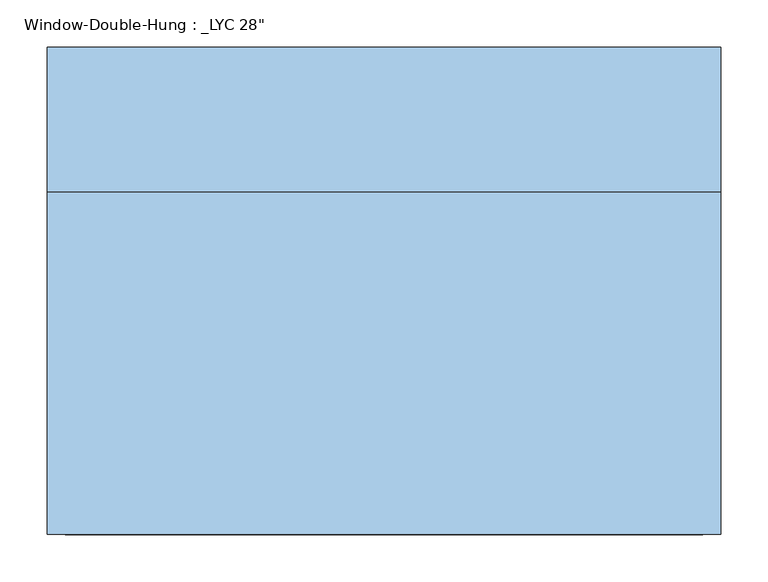
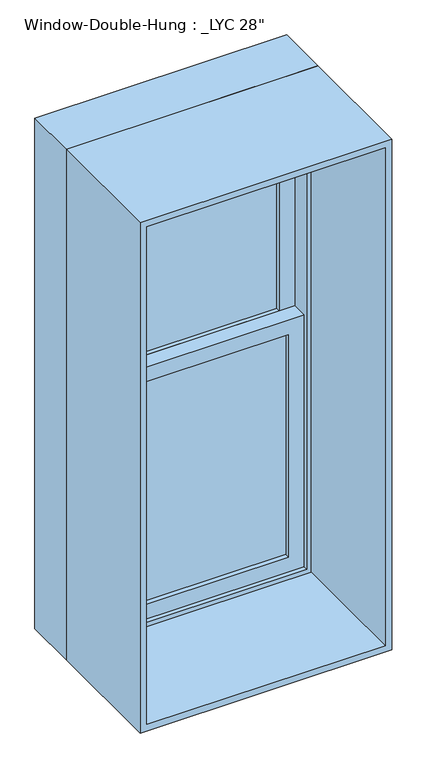
"""IFC4 building model written with IfcOpenShell, lengths in millimetres: window geometry."""

from ifc_helpers import new_model, si_unit, frame, origin, place, context, project, spatial, polyline, outline, extrude, source, transform, mapped, element, save


def window_246d4ddb(model_context):
    return source(origin(), model_context, "Body", "SweptSolid", [
        extrude(outline(polyline([(279.4, 158.75), (279.4, 152.4), (-279.4, 152.4), (-279.4, 158.75), (279.4, 158.75)])), frame((0.0, 0.0, 990.6), z_axis=(0.0, 0.0, 1.0), x_axis=(1.0, 0.0, 0.0)), (0.0, 0.0, 1.0), 663.575),
        extrude(outline(polyline([(-279.4, 146.05), (279.4, 146.05), (279.4, 139.7), (-279.4, 139.7), (-279.4, 146.05)])), frame((0.0, 0.0, 990.6), z_axis=(0.0, 0.0, 1.0), x_axis=(1.0, 0.0, 0.0)), (0.0, 0.0, 1.0), 663.575),
        extrude(outline(polyline([(279.4, 203.2), (279.4, 196.85), (-279.4, 196.85), (-279.4, 203.2), (279.4, 203.2)])), frame((0.0, 0.0, 1698.625), z_axis=(0.0, 0.0, 1.0), x_axis=(1.0, 0.0, 0.0)), (0.0, 0.0, 1.0), 663.575),
        extrude(outline(polyline([(-279.4, 190.5), (279.4, 190.5), (279.4, 184.15), (-279.4, 184.15), (-279.4, 190.5)])), frame((0.0, 0.0, 1698.625), z_axis=(0.0, 0.0, 1.0), x_axis=(1.0, 0.0, 0.0)), (0.0, 0.0, 1.0), 663.575),
        extrude(outline(polyline([(1698.625, -323.85), (946.15, -323.85), (946.15, 323.85), (1698.625, 323.85), (1698.625, -323.85)]), holes=[polyline([(1654.175, 279.4), (990.6, 279.4), (990.6, -279.4), (1654.175, -279.4), (1654.175, 279.4)])]), frame((0.0, 127.0, 0.0), z_axis=(0.0, 1.0, 0.0), x_axis=(0.0, 0.0, 1.0)), (0.0, 0.0, 1.0), 44.45),
        extrude(outline(polyline([(2406.65, -323.85), (1654.175, -323.85), (1654.175, 323.85), (2406.65, 323.85), (2406.65, -323.85)]), holes=[polyline([(2362.2, 279.4), (1698.625, 279.4), (1698.625, -279.4), (2362.2, -279.4), (2362.2, 279.4)])]), frame((0.0, 171.45, 0.0), z_axis=(0.0, 1.0, 0.0), x_axis=(0.0, 0.0, 1.0)), (0.0, 0.0, 1.0), 44.45),
        extrude(outline(polyline([(2438.4, -355.6), (914.4, -355.6), (914.4, 355.6), (2438.4, 355.6), (2438.4, -355.6)]), holes=[polyline([(2406.65, 323.85), (946.15, 323.85), (946.15, -323.85), (2406.65, -323.85), (2406.65, 323.85)])]), frame((0.0, 114.3, 0.0), z_axis=(0.0, 1.0, 0.0), x_axis=(0.0, 0.0, 1.0)), (0.0, 0.0, 1.0), 152.4),
        extrude(outline(polyline([(2438.4, 355.6), (2438.4, -355.6), (914.4, -355.6), (914.4, 355.6), (2438.4, 355.6)]), holes=[polyline([(2419.35, 336.55), (933.45, 336.55), (933.45, -336.55), (2419.35, -336.55), (2419.35, 336.55)])]), frame((0.0, -247.65, 0.0), z_axis=(0.0, 1.0, 0.0), x_axis=(0.0, 0.0, 1.0)), (0.0, 0.0, 1.0), 361.95),
    ])


if __name__ == "__main__":
    model = new_model("IFC4")
    model_context = context("Model", 3, world=origin())
    ifc_project = project(units=[si_unit("LENGTHUNIT", "METRE", prefix="MILLI")], contexts=[model_context])
    site = spatial("IfcSite", under=ifc_project)
    building = spatial("IfcBuilding", under=site)
    placement = place(None, origin())
    window_shape = window_246d4ddb(model_context)
    element("IfcWindow", 1, ObjectType="Window-Double-Hung : _LYC 28\"", at=placement, inside=building, context=model_context, shape_type="MappedRepresentation", body=[
        mapped(window_shape, transform((0.0, 0.0, 0.0), x_axis=(1.0, 0.0, 0.0), y_axis=(0.0, 1.0, 0.0), z_axis=(0.0, 0.0, 1.0))),
    ])
    save(model, "model.ifc")

# Revit data of these elements
# Type "Window-Double-Hung : _LYC 28\""
#   Type Mark = "22"
#   Fire Rating = "0.5h"
#   Assembly Code = "B2020100"
#   Wall Thickness [instance default] = 0' - 6"
#   Visual Light Transmittance = 0.9
#   Thermal Resistance (R) = 1.8146 (h·ft²·°F)/BTU
#   Solar Heat Gain Coefficient = 0.78
#   Rough Width = 2' - 4 1/2"
#   Rough Height = 5' - 0 1/2"
#   Muntin Width = 1' - 10"
#   Muntin Height = 2' - 2 1/8"
#   Interior Wall Closure [instance default] = 0' - 1 1/2"
#   Heat Transfer Coefficient (U) = 0.6496 BTU/(h·ft²·°F)
#   Frame Extension [instance default] = 0' - 2"
#   Exterior Wall Closure [instance default] = 0' - 0 1/2"
#   Extension Jamb [instance default] = 0' - 0 3/4"
#   Height = 5' - 0"
#   Width = 2' - 4"
#   Window Inset [instance default] = 0' - 0 3/4"
#   Top Muntin Visibility = yes
#   Interior Trim Visibility [instance default] = yes
#   Indicator Visibility [instance default] = yes
#   Exterior Trim Visibility [instance default] = yes
#   Extension Jamb Visibility [instance default] = yes
#   Define Thermal Properties by = 1
#   Bottom Muntin Visibility = yes
#   Muntin Pattern = Muntin Pattern_2x2 : Muntin Pattern_2x2
#   Interior Trim Material = Wood - Stained
#   Interior Trim = Trim-Window-Interior-Flat : Picture Frame
#   Interior Frame Material = Wood - Stained
#   Glass Panel Material = Glass
#   Exterior Trim Material = Clad - White
#   Exterior Trim = Trim-Window-Exterior-Flat : with Sill
#   Exterior Frame Material = Clad - White
#   Construction Type Id = ""
#   Wall Closure = (empty or 0)
#   Analytic Construction = (empty or 0)
# Element 1 (IfcWindow, "Window-Double-Hung : _LYC 28\"")
#   Wall Thickness = 1' - 7 1/2"
#   Extension Jamb = 1' - 2 1/4"
#   Materials on its faces: "Wood - Stained", "Glass", "Clad - White"
# Materials
#   "Wood - Stained": class "Wood", colour RGB 224 178 126, transparency 0, Cost = 0
#   "Glass": class "Unassigned", colour RGB 0 128 192, transparency 0.75
#   "Clad - White": class "Wood", colour RGB 242 242 238, transparency 0, Cost = 0
